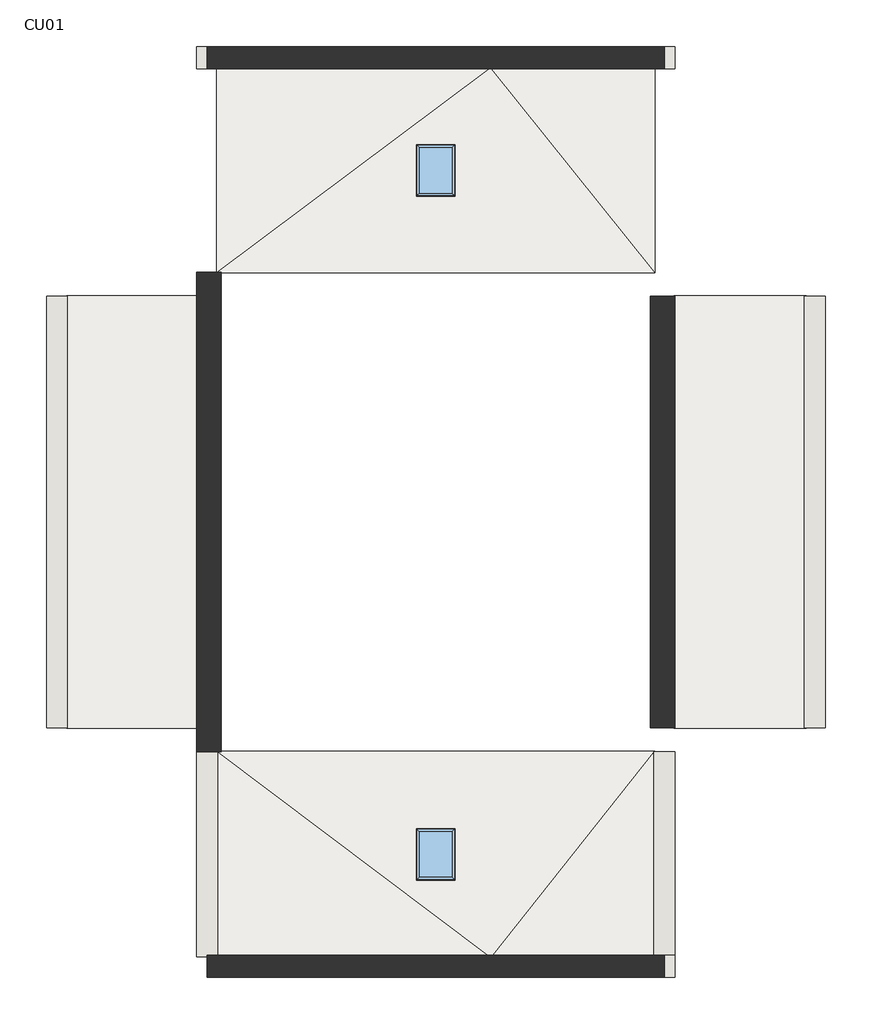
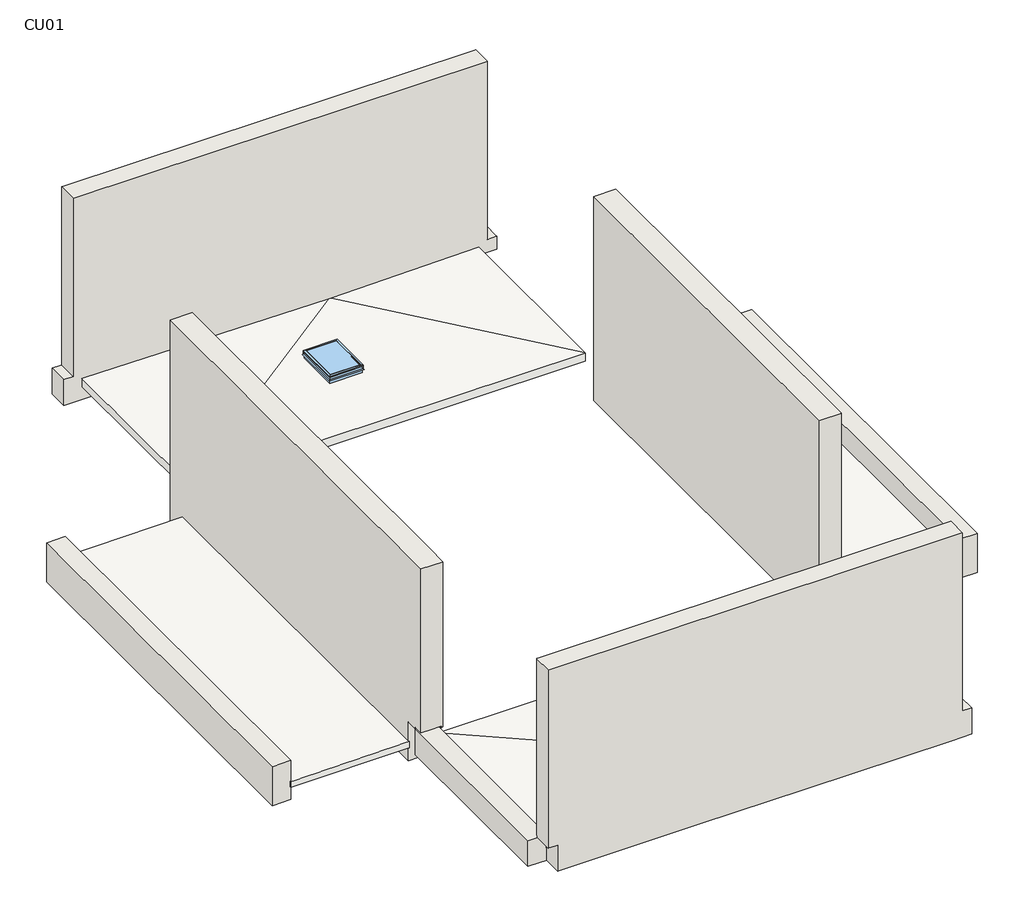
# One storey: 8 walls, 4 roofs, 2 windows.
"""IFC4 building model written with IfcOpenShell, lengths in millimetres."""

import ifcopenshell
import ifcopenshell.guid

model = None  # the IFC model being written
_history = None  # IfcOwnerHistory: only IFC2X3 demands one
_inside = {}  # id of a spatial element -> (the spatial element, [elements in it])
_under = {}  # id of a project, library or spatial element -> (it, [spatial elements below it])
_declared = {}  # id of a project -> (the project, [libraries it declares])
_typed = {}  # id of a type object -> (the type object, [elements of that type])
_made_of = {}  # id of a material, layer set ... -> (it, [elements and type objects made of it])


def new_model(schema):
    """Start an empty IFC model of exactly this schema.

    Asked for "IFC4X3", IfcOpenShell would pick the latest addendum, in which some entities
    have other attributes; the version numbers below select the first issue.
    IFC2X3 requires an IfcOwnerHistory on every rooted entity: one is made here for all.
    """
    global model, _history
    if schema == "IFC4X3":
        model = ifcopenshell.file(schema_version=(4, 3, 0, 0))
    else:
        model = ifcopenshell.file(schema=schema)
    _inside.clear()
    _under.clear()
    _declared.clear()
    _typed.clear()
    _made_of.clear()
    _history = None
    if model.schema == "IFC2X3":
        org = make("IfcOrganization", Name="unknown")
        user = make(
            "IfcPersonAndOrganization",
            ThePerson=make("IfcPerson", FamilyName="unknown"),
            TheOrganization=org,
        )
        app = make(
            "IfcApplication",
            ApplicationDeveloper=org,
            Version="unknown",
            ApplicationFullName="unknown",
            ApplicationIdentifier="unknown",
        )
        _history = make(
            "IfcOwnerHistory",
            OwningUser=user,
            OwningApplication=app,
            ChangeAction="ADDED",
            CreationDate=0,
        )
    return model


def make(cls, **values):
    """One entity of the class cls with the attributes given. An attribute that is None is left unset."""
    return model.create_entity(
        cls, **{name: value for name, value in values.items() if value is not None}
    )


def rooted(cls, **values):
    """An entity with a GlobalId (a new one), such as an element, a storey or a relation."""
    return make(cls, GlobalId=ifcopenshell.guid.new(), OwnerHistory=_history, **values)


def si_unit(unit_type, name, prefix=None):
    """IfcSIUnit, for example si_unit("LENGTHUNIT", "METRE", prefix="MILLI")."""
    return make("IfcSIUnit", UnitType=unit_type, Prefix=prefix, Name=name)


def assignment(units):
    """IfcUnitAssignment: the units of a project."""
    return None if units is None else make("IfcUnitAssignment", Units=units)


def point(xyz):
    """IfcCartesianPoint."""
    return None if xyz is None else make("IfcCartesianPoint", Coordinates=xyz)


def direction(xyz):
    """IfcDirection."""
    return None if xyz is None else make("IfcDirection", DirectionRatios=xyz)


def frame(location, z_axis=None, x_axis=None):
    """IfcAxis2Placement3D, a coordinate frame: its origin and axes. An axis left out is left unset."""
    return make(
        "IfcAxis2Placement3D",
        Location=point(location),
        Axis=direction(z_axis),
        RefDirection=direction(x_axis),
    )


def origin():
    """The frame at (0, 0, 0) with its axes left unset."""
    return frame((0.0, 0.0, 0.0))


def place(relative_to, where):
    """IfcLocalPlacement: puts the frame where relative to a parent placement (None: the world)."""
    return make(
        "IfcLocalPlacement", PlacementRelTo=relative_to, RelativePlacement=where
    )


def context(
    kind, dimensions, precision=None, world=None, true_north=None, identifier=None
):
    """IfcGeometricRepresentationContext, for example the 3D "Model" context."""
    return make(
        "IfcGeometricRepresentationContext",
        ContextIdentifier=identifier,
        ContextType=kind,
        CoordinateSpaceDimension=dimensions,
        Precision=precision,
        WorldCoordinateSystem=world,
        TrueNorth=true_north,
    )


def project(units=None, contexts=None):
    """IfcProject with its units and contexts."""
    return rooted(
        "IfcProject",
        Name="project",
        RepresentationContexts=contexts,
        UnitsInContext=assignment(units),
    )


def spatial(cls, under=None, at=None, **own):
    """A site, building, storey or space (cls), placed at a placement, below another one or the project."""
    s = rooted(cls, ObjectPlacement=at, **own)
    if under is not None:
        _under.setdefault(under.id(), (under, []))[1].append(s)
    return s


def polyline(points):
    """IfcPolyline through the points."""
    return make("IfcPolyline", Points=[point(p) for p in points])


def circle_curve(where, radius):
    """IfcCircle in the frame where."""
    return make("IfcCircle", Position=where, Radius=radius)


def outline(outer, holes=None, kind="AREA"):
    """IfcArbitraryClosedProfileDef: a profile drawn as a closed curve; with holes, ...WithVoids."""
    if holes is None:
        return make("IfcArbitraryClosedProfileDef", ProfileType=kind, OuterCurve=outer)
    return make(
        "IfcArbitraryProfileDefWithVoids",
        ProfileType=kind,
        OuterCurve=outer,
        InnerCurves=holes,
    )


def extrude(swept, where, along, depth):
    """IfcExtrudedAreaSolid: the profile swept, set in the frame where, extruded along a direction by depth."""
    return make(
        "IfcExtrudedAreaSolid",
        SweptArea=swept,
        Position=where,
        ExtrudedDirection=direction(along),
        Depth=depth,
    )


def faces_of(points, faces, orient=None, outer=None):
    """IfcFace entities. A face is a list of loops; a loop is a list of indices into points, from 0.

    orient and outer hold one flag for each loop. By default every Orientation is true, the
    first loop of a face is its IfcFaceOuterBound and the others are IfcFaceBound.
    """
    made = []
    for i, loops in enumerate(faces):
        bounds = []
        for j, loop in enumerate(loops):
            is_outer = j == 0 if outer is None else outer[i][j]
            bounds.append(
                make(
                    "IfcFaceOuterBound" if is_outer else "IfcFaceBound",
                    Bound=make("IfcPolyLoop", Polygon=[points[k] for k in loop]),
                    Orientation=True if orient is None else orient[i][j],
                )
            )
        made.append(make("IfcFace", Bounds=bounds))
    return made


def faceted_brep(points, faces, orient=None, outer=None, voids=None):
    """IfcFacetedBrep: a solid bounded by flat faces; with voids (closed shells), ...WithVoids."""
    shared = [point(p) for p in points]
    hull = make("IfcClosedShell", CfsFaces=faces_of(shared, faces, orient, outer))
    if voids is None:
        return make("IfcFacetedBrep", Outer=hull)
    return make(
        "IfcFacetedBrepWithVoids",
        Outer=hull,
        Voids=[
            make(cls, CfsFaces=faces_of(shared, fs, o, b)) for cls, fs, o, b in voids
        ],
    )


def shape(context_of_items, identifier, shape_type, items):
    """IfcShapeRepresentation: the items that make up one representation, for example the "Body"."""
    return make(
        "IfcShapeRepresentation",
        ContextOfItems=context_of_items,
        RepresentationIdentifier=identifier,
        RepresentationType=shape_type,
        Items=items,
    )


def source(mapping_origin, context_of_items, identifier, shape_type, items):
    """IfcRepresentationMap: a shape defined once, which mapped items show again and again."""
    return make(
        "IfcRepresentationMap",
        MappingOrigin=mapping_origin,
        MappedRepresentation=shape(context_of_items, identifier, shape_type, items),
    )


def transform(
    local_origin,
    x_axis=None,
    y_axis=None,
    z_axis=None,
    scale=None,
    scale2=None,
    scale3=None,
    uniform=True,
):
    """IfcCartesianTransformationOperator3D, or its non-uniform kind. x_axis, y_axis, z_axis: its Axis1, 2, 3."""
    if uniform:
        return make(
            "IfcCartesianTransformationOperator3D",
            Axis1=direction(x_axis),
            Axis2=direction(y_axis),
            LocalOrigin=point(local_origin),
            Scale=scale,
            Axis3=direction(z_axis),
        )
    return make(
        "IfcCartesianTransformationOperator3DnonUniform",
        Axis1=direction(x_axis),
        Axis2=direction(y_axis),
        LocalOrigin=point(local_origin),
        Scale=scale,
        Axis3=direction(z_axis),
        Scale2=scale2,
        Scale3=scale3,
    )


def mapped(mapping_source, mapping_target):
    """IfcMappedItem: shows the shape of a source again, moved by a transform."""
    return make(
        "IfcMappedItem", MappingSource=mapping_source, MappingTarget=mapping_target
    )


def made_of(thing, what):
    """Note that an element or type object is made of a material, layer set ...; save() writes the relation."""
    if what is not None:
        _made_of.setdefault(what.id(), (what, []))[1].append(thing)
    return thing


def element(
    cls,
    number,
    at=None,
    inside=None,
    cuts=None,
    type_object=None,
    material=None,
    context=None,
    identifier="Body",
    shape_type=None,
    held_by="IfcProductDefinitionShape",
    body=None,
    shapes=None,
    **own,
):
    """One element of the class cls, such as IfcWall. Its Tag is "e" and its number.

    at: its placement. inside: the storey or other place that contains it. cuts: it is an
    opening in that element (IfcRelVoidsElement). A single representation is given by context,
    identifier, shape_type and body (its items); several are given by shapes. held_by: the class
    of the entity that holds the representations. save() writes the other relations.
    """
    e = rooted(cls, Tag="e%d" % number, ObjectPlacement=at, **own)
    if body is not None:
        shapes = [shape(context, identifier, shape_type, body)]
    if shapes is not None:
        e.Representation = make(held_by, Representations=shapes)
    if inside is not None:
        _inside.setdefault(inside.id(), (inside, []))[1].append(e)
    if cuts is not None:
        rooted(
            "IfcRelVoidsElement", RelatingBuildingElement=cuts, RelatedOpeningElement=e
        )
    if type_object is not None:
        _typed.setdefault(type_object.id(), (type_object, []))[1].append(e)
    return made_of(e, material)


def aggregate(whole, parts):
    """IfcRelAggregates: a whole, such as a stair, and the parts it consists of."""
    return rooted("IfcRelAggregates", RelatingObject=whole, RelatedObjects=parts)


def save(model, path):
    """Write the relations noted so far, then the file.

    IfcRelAggregates (storeys below a building ...), IfcRelContainedInSpatialStructure (elements
    in a storey), IfcRelDefinesByType, IfcRelAssociatesMaterial and IfcRelDeclares: one each for
    every whole, place, type object, material and project.
    """
    for whole, parts in _under.values():
        aggregate(whole, parts)
    for where, things in _inside.values():
        rooted(
            "IfcRelContainedInSpatialStructure",
            RelatedElements=things,
            RelatingStructure=where,
        )
    for kind, things in _typed.values():
        rooted("IfcRelDefinesByType", RelatedObjects=things, RelatingType=kind)
    for what, things in _made_of.values():
        rooted("IfcRelAssociatesMaterial", RelatedObjects=things, RelatingMaterial=what)
    for by, libraries in _declared.values():
        rooted("IfcRelDeclares", RelatingContext=by, RelatedDefinitions=libraries)
    model.write(path)


def plane_surface(at):
    """IfcPlane: the flat surface through the origin of the frame at, square to its z axis."""
    return make("IfcPlane", Position=at)


def cylinder_surface(at, radius):
    """IfcCylindricalSurface: all points at the distance radius from the z axis of the frame at."""
    return make("IfcCylindricalSurface", Position=at, Radius=radius)


def advanced_brep(points, edges, surfaces, faces):
    """IfcAdvancedBrep: a solid bounded by faces that lie on surfaces and meet in shared edges.

    An edge is (start, end): straight between two places in points (the first is 0);
    or (start, end, curve); or (start, end, curve, False) where it runs against its curve.
    A face is (place in surfaces, loops), or (place, loops, False) where it looks against
    its surface's normal. A loop lists edges by number (the first is 1), with a minus sign
    where the edge is run from its end to its start. The first loop is the outer one.
    """
    corners = [point(p) for p in points]
    vertices = [make("IfcVertexPoint", VertexGeometry=c) for c in corners]
    made = []
    for start, end, *more in edges:
        made.append(
            make(
                "IfcEdgeCurve",
                EdgeStart=vertices[start],
                EdgeEnd=vertices[end],
                EdgeGeometry=more[0] if more else make("IfcPolyline", Points=[corners[start], corners[end]]),
                SameSense=more[1] if len(more) > 1 else True,
            )
        )
    hull = []
    for where, loops, *sense in faces:
        bounds = []
        for j, loop in enumerate(loops):
            ring = [make("IfcOrientedEdge", EdgeElement=made[abs(k) - 1], Orientation=k > 0) for k in loop]
            bounds.append(
                make(
                    "IfcFaceOuterBound" if j == 0 else "IfcFaceBound",
                    Bound=make("IfcEdgeLoop", EdgeList=ring),
                    Orientation=True,
                )
            )
        hull.append(make("IfcAdvancedFace", Bounds=bounds, FaceSurface=surfaces[where], SameSense=sense[0] if sense else True))
    return make("IfcAdvancedBrep", Outer=make("IfcClosedShell", CfsFaces=hull))


def claraboya_0711_x_0965mm_26b2130f(model_context):
    return source(origin(), model_context, "Body", "SolidModel", [
        faceted_brep([(254.440073, 370.1040988, 4001.2), (279.840073, 395.5040988, 4001.2), (279.840073, -569.4959012, 4001.2), (254.440073, -544.0959012, 4001.2), (254.440073, 370.1040988, 4026.6), (254.440073, -544.0959012, 4026.6), (292.540073, 408.2040988, 4026.6), (292.540073, -582.1959012, 4026.6), (292.540073, 408.2040988, 4001.2), (292.540073, -582.1959012, 4001.2), (292.540073, 408.2040988, 3950.4), (292.540073, -582.1959012, 3950.4), (307.1089145, 422.7729403, 3929.5935381), (307.1089145, -596.7647427, 3929.5935381), (301.907299, 417.5713248, 3925.9513277), (301.907299, -591.5631272, 3925.9513277), (286.190073, 401.8540988, 3948.3978527), (286.190073, -575.8459012, 3948.3978527), (286.190073, 401.8540988, 4001.2), (286.190073, -575.8459012, 4001.2), (-431.159927, -569.4959012, 4001.2), (-405.759927, -544.0959012, 4001.2), (-405.759927, -544.0959012, 4026.6), (-443.859927, -582.1959012, 4026.6), (-443.859927, -582.1959012, 4001.2), (-443.859927, -582.1959012, 3950.4), (-458.4287685, -596.7647427, 3929.5935381), (-453.227153, -591.5631272, 3925.9513277), (-437.509927, -575.8459012, 3948.3978527), (-437.509927, -575.8459012, 4001.2), (-431.159927, 395.5040988, 4001.2), (-405.759927, 370.1040988, 4001.2), (-405.759927, 370.1040988, 4026.6), (-443.859927, 408.2040988, 4026.6), (-443.859927, 408.2040988, 4001.2), (-443.859927, 408.2040988, 3950.4), (-458.4287685, 422.7729403, 3929.5935381), (-453.227153, 417.5713248, 3925.9513277), (-437.509927, 401.8540988, 3948.3978527), (-437.509927, 401.8540988, 4001.2)], [[[0, 1, 2, 3]], [[4, 0, 3, 5]], [[6, 4, 5, 7]], [[8, 6, 7, 9]], [[10, 8, 9, 11]], [[12, 10, 11, 13]], [[14, 12, 13, 15]], [[16, 14, 15, 17]], [[18, 16, 17, 19]], [[1, 18, 19, 2]], [[3, 2, 20, 21]], [[5, 3, 21, 22]], [[7, 5, 22, 23]], [[9, 7, 23, 24]], [[11, 9, 24, 25]], [[13, 11, 25, 26]], [[15, 13, 26, 27]], [[17, 15, 27, 28]], [[19, 17, 28, 29]], [[2, 19, 29, 20]], [[21, 20, 30, 31]], [[22, 21, 31, 32]], [[23, 22, 32, 33]], [[24, 23, 33, 34]], [[25, 24, 34, 35]], [[26, 25, 35, 36]], [[27, 26, 36, 37]], [[28, 27, 37, 38]], [[29, 28, 38, 39]], [[20, 29, 39, 30]], [[31, 30, 1, 0]], [[32, 31, 0, 4]], [[33, 32, 4, 6]], [[34, 33, 6, 8]], [[35, 34, 8, 10]], [[36, 35, 10, 12]], [[37, 36, 12, 14]], [[38, 37, 14, 16]], [[39, 38, 16, 18]], [[30, 39, 18, 1]]]),
        faceted_brep([(279.840073, -569.4959012, 4001.2), (279.840073, -569.4959012, 3848.8), (279.840073, 395.5040988, 3848.8), (279.840073, 395.5040988, 4001.2), (254.440073, -544.0959012, 4001.2), (254.440073, 370.1040988, 4001.2), (254.440073, -544.0959012, 3975.8), (254.440073, 370.1040988, 3975.8), (235.390073, -525.0459012, 3975.8), (235.390073, 351.0540988, 3975.8), (235.390073, -525.0459012, 3848.8), (235.390073, 351.0540988, 3848.8), (-431.159927, 395.5040988, 3848.8), (-431.159927, 395.5040988, 4001.2), (-405.759927, 370.1040988, 4001.2), (-405.759927, 370.1040988, 3975.8), (-386.709927, 351.0540988, 3975.8), (-386.709927, 351.0540988, 3848.8), (-431.159927, -569.4959012, 3848.8), (-431.159927, -569.4959012, 4001.2), (-405.759927, -544.0959012, 4001.2), (-405.759927, -544.0959012, 3975.8), (-386.709927, -525.0459012, 3975.8), (-386.709927, -525.0459012, 3848.8)], [[[0, 1, 2, 3]], [[4, 0, 3, 5]], [[6, 4, 5, 7]], [[8, 6, 7, 9]], [[10, 8, 9, 11]], [[1, 10, 11, 2]], [[3, 2, 12, 13]], [[5, 3, 13, 14]], [[7, 5, 14, 15]], [[9, 7, 15, 16]], [[11, 9, 16, 17]], [[2, 11, 17, 12]], [[13, 12, 18, 19]], [[14, 13, 19, 20]], [[15, 14, 20, 21]], [[16, 15, 21, 22]], [[17, 16, 22, 23]], [[12, 17, 23, 18]], [[19, 18, 1, 0]], [[20, 19, 0, 4]], [[21, 20, 4, 6]], [[22, 21, 6, 8]], [[23, 22, 8, 10]], [[18, 23, 10, 1]]]),
        extrude(outline(polyline([(254.440073, -544.0959012), (-405.759927, -544.0959012), (-405.759927, 370.1040988), (254.440073, 370.1040988), (254.440073, -544.0959012)])), frame((0.0, 0.0, 4020.25), z_axis=(0.0, 0.0, 1.0), x_axis=(1.0, 0.0, 0.0)), (0.0, 0.0, 1.0), 6.35),
    ])


def claraboya_0711_x_0965mm_17ef4467(model_context):
    return source(origin(), model_context, "Body", "SolidModel", [
        faceted_brep([(254.440073, -370.1040988, 4001.2), (254.440073, 544.0959012, 4001.2), (279.840073, 569.4959012, 4001.2), (279.840073, -395.5040988, 4001.2), (254.440073, -370.1040988, 4026.6), (254.440073, 544.0959012, 4026.6), (292.540073, -408.2040988, 4026.6), (292.540073, 582.1959012, 4026.6), (292.540073, -408.2040988, 4001.2), (292.540073, 582.1959012, 4001.2), (292.540073, -408.2040988, 3950.4), (292.540073, 582.1959012, 3950.4), (307.1089145, -422.7729403, 3929.5935381), (307.1089145, 596.7647427, 3929.5935381), (301.907299, -417.5713248, 3925.9513277), (301.907299, 591.5631272, 3925.9513277), (286.190073, -401.8540988, 3948.3978527), (286.190073, 575.8459012, 3948.3978527), (286.190073, -401.8540988, 4001.2), (286.190073, 575.8459012, 4001.2), (-405.759927, 544.0959012, 4001.2), (-431.159927, 569.4959012, 4001.2), (-405.759927, 544.0959012, 4026.6), (-443.859927, 582.1959012, 4026.6), (-443.859927, 582.1959012, 4001.2), (-443.859927, 582.1959012, 3950.4), (-458.4287685, 596.7647427, 3929.5935381), (-453.227153, 591.5631272, 3925.9513277), (-437.509927, 575.8459012, 3948.3978527), (-437.509927, 575.8459012, 4001.2), (-405.759927, -370.1040988, 4001.2), (-431.159927, -395.5040988, 4001.2), (-405.759927, -370.1040988, 4026.6), (-443.859927, -408.2040988, 4026.6), (-443.859927, -408.2040988, 4001.2), (-443.859927, -408.2040988, 3950.4), (-458.4287685, -422.7729403, 3929.5935381), (-453.227153, -417.5713248, 3925.9513277), (-437.509927, -401.8540988, 3948.3978527), (-437.509927, -401.8540988, 4001.2)], [[[0, 1, 2, 3]], [[4, 5, 1, 0]], [[6, 7, 5, 4]], [[8, 9, 7, 6]], [[10, 11, 9, 8]], [[12, 13, 11, 10]], [[14, 15, 13, 12]], [[16, 17, 15, 14]], [[18, 19, 17, 16]], [[3, 2, 19, 18]], [[1, 20, 21, 2]], [[5, 22, 20, 1]], [[7, 23, 22, 5]], [[9, 24, 23, 7]], [[11, 25, 24, 9]], [[13, 26, 25, 11]], [[15, 27, 26, 13]], [[17, 28, 27, 15]], [[19, 29, 28, 17]], [[2, 21, 29, 19]], [[20, 30, 31, 21]], [[22, 32, 30, 20]], [[23, 33, 32, 22]], [[24, 34, 33, 23]], [[25, 35, 34, 24]], [[26, 36, 35, 25]], [[27, 37, 36, 26]], [[28, 38, 37, 27]], [[29, 39, 38, 28]], [[21, 31, 39, 29]], [[30, 0, 3, 31]], [[32, 4, 0, 30]], [[33, 6, 4, 32]], [[34, 8, 6, 33]], [[35, 10, 8, 34]], [[36, 12, 10, 35]], [[37, 14, 12, 36]], [[38, 16, 14, 37]], [[39, 18, 16, 38]], [[31, 3, 18, 39]]]),
        faceted_brep([(279.840073, 569.4959012, 4001.2), (279.840073, -395.5040988, 4001.2), (279.840073, -395.5040988, 3848.8), (279.840073, 569.4959012, 3848.8), (254.440073, 544.0959012, 4001.2), (254.440073, -370.1040988, 4001.2), (254.440073, 544.0959012, 3975.8), (254.440073, -370.1040988, 3975.8), (235.390073, 525.0459012, 3975.8), (235.390073, -351.0540988, 3975.8), (235.390073, 525.0459012, 3848.8), (235.390073, -351.0540988, 3848.8), (-431.159927, -395.5040988, 4001.2), (-431.159927, -395.5040988, 3848.8), (-405.759927, -370.1040988, 4001.2), (-405.759927, -370.1040988, 3975.8), (-386.709927, -351.0540988, 3975.8), (-386.709927, -351.0540988, 3848.8), (-431.159927, 569.4959012, 4001.2), (-431.159927, 569.4959012, 3848.8), (-405.759927, 544.0959012, 4001.2), (-405.759927, 544.0959012, 3975.8), (-386.709927, 525.0459012, 3975.8), (-386.709927, 525.0459012, 3848.8)], [[[0, 1, 2, 3]], [[4, 5, 1, 0]], [[6, 7, 5, 4]], [[8, 9, 7, 6]], [[10, 11, 9, 8]], [[3, 2, 11, 10]], [[1, 12, 13, 2]], [[5, 14, 12, 1]], [[7, 15, 14, 5]], [[9, 16, 15, 7]], [[11, 17, 16, 9]], [[2, 13, 17, 11]], [[12, 18, 19, 13]], [[14, 20, 18, 12]], [[15, 21, 20, 14]], [[16, 22, 21, 15]], [[17, 23, 22, 16]], [[13, 19, 23, 17]], [[18, 0, 3, 19]], [[20, 4, 0, 18]], [[21, 6, 4, 20]], [[22, 8, 6, 21]], [[23, 10, 8, 22]], [[19, 3, 10, 23]]]),
        extrude(outline(polyline([(254.440073, 544.0959012), (254.440073, -370.1040988), (-405.759927, -370.1040988), (-405.759927, 544.0959012), (254.440073, 544.0959012)])), frame((0.0, 0.0, 4020.25), z_axis=(0.0, 0.0, 1.0), x_axis=(1.0, 0.0, 0.0)), (0.0, 0.0, 1.0), 6.35),
    ])


model = new_model("IFC4")

# Units and contexts
model_context = context("Model", 3, world=origin())
ifc_project = project(units=[si_unit("LENGTHUNIT", "METRE", prefix="MILLI")], contexts=[model_context])

# Site, building, storey
site = spatial("IfcSite", under=ifc_project)
building = spatial("IfcBuilding", under=site)
storey = spatial("IfcBuildingStorey", under=building, Name="CU01", Elevation=2430.0)

# Roofs
placement = place(None, origin())
element("IfcRoof", 1, ObjectType="ACAB CUB GRAVA INF-A_PABLO", at=placement, inside=storey, context=model_context, shape_type="Brep", body=[
    faceted_brep([(-12165.0, -4267.5, 2730.0), (-12165.0, -4252.5, 2730.0), (-12165.0, -232.5, 2730.0), (-12165.0, -217.5, 2730.0), (-12165.0, -217.5, 2921.2), (-12165.0, -232.5, 2921.2), (-12165.0, -4252.5, 2921.2), (-12165.0, -4267.5, 2921.2), (-12235.0, -217.5, 2730.0), (-20835.0, -217.5, 2730.0), (-20835.0, -217.5, 2921.2), (-15415.0, -217.5, 2871.2), (-16188.95, -1804.45, 2890.7919753), (-16188.95, -1804.45, 2730.0), (-16188.95, -2680.55, 2730.0), (-16188.95, -2680.55, 2901.6080247), (-16811.05, -2680.55, 2730.0), (-16811.05, -2680.55, 2901.6080247), (-16811.05, -1804.45, 2730.0), (-16811.05, -1804.45, 2890.7919753), (-20750.0, -4267.5, 2730.0), (-20835.0, -4267.5, 2730.0), (-20835.0, -4252.5, 2730.0), (-20835.0, -232.5, 2730.0), (-20835.0, -4267.5, 2921.2), (-20835.0, -4252.5, 2921.2), (-20835.0, -232.5, 2921.2), (-20750.0, -4267.5, 2921.2), (-12177.037037, -4252.5, 2921.0148148), (-12180.0, -4248.8076923, 2920.9692308), (-15402.962963, -232.5, 2871.3851852), (-15435.0740741, -232.5, 2871.3851852)], [[[0, 1, 2, 3, 4, 5, 6, 7]], [[3, 8, 9, 10, 11, 4]], [[12, 13, 14, 15]], [[15, 14, 16, 17]], [[17, 16, 18, 19]], [[13, 12, 19, 18]], [[3, 2, 1, 0, 20, 21, 22, 23, 9, 8], [14, 13, 18, 16]], [[9, 23, 22, 21, 24, 25, 26, 10]], [[0, 7, 27, 24, 21, 20]], [[24, 27, 7, 28, 29, 30, 11, 31], [12, 15, 17, 19]], [[7, 6, 5, 4, 11, 30, 29, 28]], [[10, 26, 25, 24, 31, 11]]]),
])
element("IfcRoof", 2, ObjectType="ACAB CUB GRAVA INF-B_PABLO", at=placement, inside=storey, context=model_context, shape_type="Brep", body=[
    faceted_brep([(-23810.0, -4717.5, 2430.0), (-21230.0, -4717.5, 2430.0), (-21215.0, -4717.5, 2430.0), (-21215.0, -13267.5, 2430.0), (-21215.0, -13282.5, 2430.0), (-21230.0, -13282.5, 2430.0), (-23810.0, -13282.5, 2430.0), (-23810.0, -13267.5, 2430.0), (-23810.0, -4732.5, 2430.0), (-21215.0, -4717.5, 2581.2), (-23810.0, -4717.5, 2551.2), (-21230.0, -4717.5, 2581.0265896), (-23810.0, -13282.5, 2551.2), (-23810.0, -13267.5, 2551.2), (-23810.0, -9000.0, 2551.2), (-23810.0, -4732.5, 2551.2), (-21215.0, -13282.5, 2581.2), (-21215.0, -13267.5, 2581.2)], [[[0, 1, 2, 3, 4, 5, 6, 7, 8]], [[9, 2, 1, 0, 10, 11]], [[10, 0, 8, 7, 6, 12, 13, 14, 15]], [[12, 6, 5, 4, 16]], [[10, 15, 14, 13, 12, 16, 17, 9, 11]], [[16, 4, 3, 2, 9, 17]]]),
])
element("IfcRoof", 3, ObjectType="ACAB CUB GRAVA INF-A_PABLO", at=placement, inside=storey, context=model_context, shape_type="Brep", body=[
    faceted_brep([(-12165.0, -17812.5, 2730.0), (-12165.0, -17767.5, 2730.0), (-12165.0, -13747.5, 2730.0), (-12165.0, -13732.5, 2730.0), (-12165.0, -13732.5, 2921.2), (-12165.0, -13747.5, 2921.2), (-12165.0, -17767.5, 2921.2), (-12165.0, -17812.5, 2921.2), (-15405.0, -17812.5, 2871.2), (-20820.0, -17812.5, 2921.0618785), (-20835.0, -17812.5, 2921.2), (-20835.0, -17812.5, 2730.0), (-20820.0, -17812.5, 2730.0), (-16188.95, -16210.55, 2730.0), (-16188.95, -16210.55, 2890.8317402), (-16188.95, -15334.45, 2901.5682598), (-16188.95, -15334.45, 2730.0), (-16811.05, -15334.45, 2901.5682598), (-16811.05, -15334.45, 2730.0), (-16811.05, -16210.55, 2890.8317402), (-16811.05, -16210.55, 2730.0), (-20835.0, -17797.5, 2730.0), (-20835.0, -13732.5, 2730.0), (-20820.0, -13732.5, 2730.0), (-20750.0, -13732.5, 2730.0), (-20835.0, -17797.5, 2921.2), (-20835.0, -13732.5, 2921.2), (-20820.0, -13732.5, 2921.2), (-20750.0, -13732.5, 2921.2), (-12176.9117647, -13747.5, 2921.0161765), (-12180.0, -13751.3888889, 2920.9685185), (-15369.2647059, -17767.5, 2871.7514706), (-20820.0, -13743.7707182, 2921.0618785), (-15464.8897059, -17767.5, 2871.7514706)], [[[0, 1, 2, 3, 4, 5, 6, 7]], [[0, 7, 8, 9, 10, 11, 12]], [[13, 14, 15, 16]], [[16, 15, 17, 18]], [[18, 17, 19, 20]], [[14, 13, 20, 19]], [[3, 2, 1, 0, 12, 11, 21, 22, 23, 24], [13, 16, 18, 20]], [[22, 21, 11, 10, 25, 26]], [[4, 3, 24, 23, 22, 26, 27, 28]], [[7, 6, 5, 4, 29, 30, 31, 8]], [[4, 28, 27, 26, 32, 33, 8, 31, 30, 29], [15, 14, 19, 17]], [[26, 25, 10, 9, 8, 33, 32]]]),
])
element("IfcRoof", 4, ObjectType="ACAB CUB GRAVA INF-B_PABLO", at=placement, inside=storey, context=model_context, shape_type="Brep", body=[
    faceted_brep([(-11785.0, -4717.5, 2430.0), (-9165.0, -4717.5, 2430.0), (-9165.0, -4732.5, 2430.0), (-9165.0, -13267.5, 2430.0), (-9165.0, -13282.5, 2430.0), (-11785.0, -13282.5, 2430.0), (-11785.0, -13267.5, 2430.0), (-11785.0, -4732.5, 2430.0), (-9165.0, -4717.5, 2551.2), (-11785.0, -4717.5, 2581.2), (-9165.0, -13282.5, 2551.2), (-9165.0, -4732.5, 2551.2), (-9165.0, -9000.0, 2551.2), (-9165.0, -13267.5, 2551.2), (-11785.0, -13282.5, 2581.2), (-11785.0, -4732.5, 2581.2), (-11785.0, -13267.5, 2581.2)], [[[0, 1, 2, 3, 4, 5, 6, 7]], [[8, 1, 0, 9]], [[10, 4, 3, 2, 1, 8, 11, 12, 13]], [[14, 5, 4, 10]], [[12, 11, 8, 9, 15, 16, 14, 10, 13]], [[9, 0, 7, 6, 5, 14, 16, 15]]]),
])

# Walls
element("IfcWall", 5, ObjectType="MURO TIPO 1_EXTERIOR_PETO_PABLO", at=placement, inside=storey, context=model_context, shape_type="Brep", body=[
    faceted_brep([(-23795.0, -13267.5, 2130.0), (-23795.0, -4732.5, 2130.0), (-23795.0, -4732.5, 2430.0), (-23795.0, -13267.5, 2430.0), (-23795.0, -4732.5, 3030.0), (-23795.0, -13267.5, 3030.0), (-23795.0, -13267.5, 2551.3734104), (-23795.0, -4732.5, 2551.3734104), (-24205.0, -4732.5, 2130.0), (-24205.0, -13267.5, 2130.0), (-24205.0, -13267.5, 3030.0), (-24205.0, -4732.5, 3030.0), (-23810.0, -13267.5, 2430.0), (-23810.0, -13267.5, 2551.2), (-23810.0, -4732.5, 2551.2), (-23810.0, -4732.5, 2430.0), (-23810.0, -9000.0, 2551.2)], [[[0, 1, 2, 3]], [[4, 5, 6, 7]], [[8, 9, 10, 11]], [[1, 0, 9, 8]], [[5, 4, 11, 10]], [[5, 10, 9, 0, 3, 12, 13, 6]], [[1, 8, 11, 4, 7, 14, 15, 2]], [[15, 12, 3, 2]], [[12, 15, 14, 16, 13]], [[13, 16, 14, 7, 6]]]),
])
element("IfcWall", 6, ObjectType="MURO TIPO 1_EXTERIOR_PETO_PABLO", at=placement, inside=storey, context=model_context, shape_type="Brep", body=[
    faceted_brep([(-8795.0, -13267.5, 2130.0), (-8795.0, -4732.5, 2130.0), (-8795.0, -4732.5, 3030.0), (-8795.0, -13267.5, 3030.0), (-9205.0, -4732.5, 2130.0), (-9205.0, -13267.5, 2130.0), (-9205.0, -13267.5, 2430.0), (-9205.0, -4732.5, 2430.0), (-9205.0, -13267.5, 3030.0), (-9205.0, -4732.5, 3030.0), (-9205.0, -4732.5, 2551.6580153), (-9205.0, -13267.5, 2551.6580153), (-9165.0, -13267.5, 2551.2), (-9165.0, -13267.5, 2430.0), (-9165.0, -4732.5, 2430.0), (-9165.0, -4732.5, 2551.2), (-9165.0, -9000.0, 2551.2)], [[[0, 1, 2, 3]], [[4, 5, 6, 7]], [[8, 9, 10, 11]], [[1, 0, 5, 4]], [[3, 2, 9, 8]], [[0, 3, 8, 11, 12, 13, 6, 5]], [[2, 1, 4, 7, 14, 15, 10, 9]], [[13, 14, 7, 6]], [[14, 13, 12, 16, 15]], [[16, 12, 11, 10, 15]]]),
])
element("IfcWall", 7, ObjectType="MURO TIPO 1_EXTERIOR_PETO-CUB_PABLO", at=placement, inside=storey, context=model_context, shape_type="Brep", body=[
    faceted_brep([(-21230.0, -232.5, 2430.0), (-12235.0, -232.5, 2430.0), (-12235.0, -232.5, 2730.0), (-20835.0, -232.5, 2730.0), (-20835.0, -232.5, 2921.2), (-15435.0740741, -232.5, 2871.3851852), (-15402.962963, -232.5, 2871.3851852), (-12180.0, -232.5, 2920.9692308), (-12165.0, -232.5, 2921.2), (-12165.0, -232.5, 2730.0), (-11770.0, -232.5, 2730.0), (-11770.0, -232.5, 3030.0), (-11975.0, -232.5, 3030.0), (-11975.0, -232.5, 7150.0), (-12002.5, -232.5, 7150.0), (-21010.0, -232.5, 7150.0), (-21025.0, -232.5, 7150.0), (-21025.0, -232.5, 3030.0), (-21230.0, -232.5, 3030.0), (-21230.0, -232.5, 2730.0), (-12235.0, 207.5, 2430.0), (-17710.0, 207.5, 2430.0), (-21230.0, 207.5, 2430.0), (-21230.0, 207.5, 3030.0), (-21025.0, 207.5, 3030.0), (-21025.0, 207.5, 7150.0), (-21010.0, 207.5, 7150.0), (-12002.5, 207.5, 7150.0), (-11975.0, 207.5, 7150.0), (-11975.0, 207.5, 3030.0), (-11770.0, 207.5, 3030.0), (-11770.0, 207.5, 2730.0), (-12235.0, 207.5, 2730.0), (-12165.0, -217.5, 2730.0), (-12235.0, -217.5, 2730.0), (-12165.0, -217.5, 2921.2), (-15415.0, -217.5, 2871.2), (-20835.0, -217.5, 2921.2), (-20835.0, -217.5, 2730.0), (-21230.0, 192.5, 3030.0), (-21230.0, -217.5, 3030.0), (-11770.0, -217.5, 3030.0), (-11770.0, 192.5, 3030.0)], [[[0, 1, 2, 3, 4, 5, 6, 7, 8, 9, 10, 11, 12, 13, 14, 15, 16, 17, 18, 19]], [[20, 21, 22, 23, 24, 25, 26, 27, 28, 29, 30, 31, 32]], [[1, 0, 22, 21, 20]], [[16, 15, 14, 13, 28, 27, 26, 25]], [[32, 31, 10, 9, 33, 34]], [[2, 1, 20, 32, 34]], [[33, 35, 36, 37, 38, 34]], [[35, 33, 9, 8]], [[34, 38, 3, 2]], [[38, 37, 4, 3]], [[16, 25, 24, 17]], [[17, 24, 23, 39, 40, 18]], [[22, 0, 19, 18, 40, 39, 23]], [[36, 35, 8, 7, 6]], [[37, 36, 5, 4]], [[36, 6, 5]], [[28, 13, 12, 29]], [[29, 12, 11, 41, 42, 30]], [[11, 10, 31, 30, 42, 41]]]),
])
element("IfcWall", 8, ObjectType="MURO TIPO 3B_ESTAR-EXT_YESO-CEMENTO_PABLO", at=placement, inside=storey, context=model_context, shape_type="Brep", body=[
    faceted_brep([(-12250.0, -4732.5, 2130.0), (-12250.0, -13267.5, 2130.0), (-12250.0, -13267.5, 6850.0), (-12250.0, -4732.5, 6850.0), (-11770.0, -13267.5, 2130.0), (-11770.0, -4732.5, 2130.0), (-11770.0, -4732.5, 2430.0), (-11770.0, -13267.5, 2430.0), (-11770.0, -4732.5, 6850.0), (-11770.0, -13267.5, 6850.0), (-11770.0, -13267.5, 2581.0282443), (-11770.0, -4732.5, 2581.0282443), (-11785.0, -13267.5, 2130.0), (-11785.0, -13267.5, 6850.0), (-11785.0, -4732.5, 2430.0), (-11785.0, -13267.5, 2430.0), (-11785.0, -13267.5, 2581.2), (-11785.0, -4732.5, 2581.2)], [[[0, 1, 2, 3]], [[4, 5, 6, 7]], [[8, 9, 10, 11]], [[1, 0, 5, 4, 12]], [[3, 2, 13, 9, 8]], [[14, 15, 7, 6]], [[16, 17, 11, 10]], [[15, 14, 17, 16]], [[1, 12, 4, 7, 15, 16, 10, 9, 13, 2]], [[5, 0, 3, 8, 11, 17, 14, 6]]]),
])
element("IfcWall", 9, ObjectType="MURO TIPO 1_EXTERIOR_PETO_PABLO", at=placement, inside=storey, context=model_context, shape_type="Brep", body=[
    faceted_brep([(-11770.0, -17767.5, 2430.0), (-11770.0, -13747.5, 2430.0), (-11770.0, -13747.5, 3030.0), (-11770.0, -17767.5, 3030.0), (-12180.0, -13747.5, 2430.0), (-12180.0, -17767.5, 2430.0), (-12180.0, -17767.5, 2730.0), (-12180.0, -13747.5, 2730.0), (-12180.0, -17767.5, 3030.0), (-12180.0, -13747.5, 3030.0), (-12180.0, -13747.5, 2921.0161765), (-12180.0, -13751.3888889, 2920.9685185), (-12180.0, -17767.5, 2920.9685185), (-11975.0, -17767.5, 3030.0), (-12165.0, -13747.5, 2921.2), (-12165.0, -13747.5, 2730.0), (-12165.0, -17767.5, 2730.0), (-12165.0, -17767.5, 2921.2), (-12176.9117647, -13747.5, 2921.0161765)], [[[0, 1, 2, 3]], [[4, 5, 6, 7]], [[8, 9, 10, 11, 12]], [[1, 0, 5, 4]], [[3, 2, 9, 8, 13]], [[14, 15, 16, 17]], [[7, 6, 16, 15]], [[11, 18, 14, 17, 12]], [[18, 11, 10]], [[2, 1, 4, 7, 15, 14, 18, 10, 9]], [[0, 3, 13, 8, 12, 17, 16, 6, 5]]]),
])
element("IfcWall", 10, ObjectType="MURO TIPO 1_EXTERIOR_PETO_PABLO", at=placement, inside=storey, context=model_context, shape_type="Brep", body=[
    faceted_brep([(-20820.0, -17797.5, 2430.0), (-20820.0, -17767.5, 2430.0), (-20820.0, -13537.5, 2430.0), (-20820.0, -13537.5, 3030.0), (-20820.0, -17767.5, 3030.0), (-20820.0, -17797.5, 3030.0), (-20820.0, -17797.5, 2921.0618785), (-20820.0, -17767.5, 2921.0618785), (-20820.0, -13743.7707182, 2921.0618785), (-20820.0, -13732.5, 2921.2), (-20820.0, -13732.5, 2730.0), (-20820.0, -17767.5, 2730.0), (-20820.0, -17797.5, 2730.0), (-21230.0, -13537.5, 2430.0), (-21230.0, -17797.5, 2430.0), (-21230.0, -17797.5, 3030.0), (-21230.0, -13537.5, 3030.0), (-21010.0, -17797.5, 3030.0), (-20835.0, -13732.5, 2730.0), (-20835.0, -17797.5, 2730.0), (-20835.0, -13732.5, 2921.2), (-20835.0, -17797.5, 2921.2)], [[[0, 1, 2, 3, 4, 5, 6, 7, 8, 9, 10, 11, 12]], [[13, 14, 15, 16]], [[2, 1, 0, 14, 13]], [[5, 4, 3, 16, 15, 17]], [[10, 18, 19, 12, 11]], [[18, 20, 21, 19]], [[20, 9, 8]], [[20, 8, 7, 6, 21]], [[3, 2, 13, 16]], [[20, 18, 10, 9]], [[5, 17, 15, 14, 0, 12, 19, 21, 6]]]),
])
element("IfcWall", 11, ObjectType="MURO TIPO 3B_ESTAR-EXT_YESO-CEMENTO_PABLO", at=placement, inside=storey, context=model_context, shape_type="AdvancedBrep", body=[
    advanced_brep(
    [(-21230.0, -4252.5, 2130.0), (-21230.0, -13267.5, 2130.0), (-21230.0, -13267.5, 2430.0), (-21230.0, -13267.5, 3030.0), (-21230.0, -13537.5, 3030.0), (-21230.0, -13537.5, 3060.7854779), (-21230.0, -13747.5, 3060.7854779), (-21230.0, -13747.5, 6850.0), (-21230.0, -4252.5, 6850.0), (-20750.0, -13267.5, 2130.0), (-20750.0, -4732.5, 2130.0), (-20750.0, -4252.5, 2130.0), (-20750.0, -4252.5, 2730.0), (-20750.0, -4252.5, 2921.0168498), (-20750.0, -4252.5, 6850.0), (-20750.0, -4732.5, 6850.0), (-20750.0, -13267.5, 6850.0), (-20750.0, -13747.5, 6850.0), (-20750.0, -13747.5, 3030.0), (-20750.0, -13537.5, 3030.0), (-20750.0, -13267.5, 3030.0), (-20750.0, -13267.5, 2430.0), (-20790.0, -13267.5, 2130.0), (-20775.0, -13537.5, 3030.0), (-20775.0, -13537.5, 3060.0), (-21025.0, -13537.5, 3064.3637662), (-20820.0, -13537.5, 3030.0), (-20804.8467624, -13537.5, 3030.0), (-20789.8467624, -13537.5, 3030.0), (-20775.0, -13747.5, 3030.0), (-20775.0, -13747.5, 3060.0), (-20804.8467624, -13747.5, 3030.0), (-20789.8467624, -13747.5, 3030.0), (-21025.0, -13747.5, 3064.3637662)],
    [
        (0, 1),
        (1, 2),
        (2, 3),
        (3, 4),
        (4, 5),
        (5, 6),
        (6, 7),
        (7, 8),
        (8, 0),
        (9, 10),
        (10, 11),
        (11, 12),
        (12, 13),
        (13, 14),
        (14, 15),
        (15, 16),
        (16, 17),
        (17, 18),
        (18, 19),
        (19, 20),
        (20, 21),
        (21, 9),
        (0, 11),
        (9, 22),
        (22, 1),
        (7, 17),
        (14, 8),
        (23, 24),
        (24, 25),
        (25, 5),
        (4, 26),
        (26, 27),
        (27, 28, circle_curve(frame((-20797.3467624, -13537.5, 3030.0), z_axis=(0.0, 1.0, 0.0), x_axis=(-1.0, 0.0, 0.0)), 7.5)),
        (28, 23),
        (23, 29),
        (29, 30),
        (30, 24),
        (27, 31),
        (31, 32, circle_curve(frame((-20797.3467624, -13747.5, 3030.0), z_axis=(0.0, 1.0, 0.0), x_axis=(-1.0, 0.0, 0.0)), 7.5)),
        (32, 28),
        (25, 33),
        (33, 6),
        (30, 33),
        (20, 3),
        (29, 18),
        (31, 32),
    ],
    [
        plane_surface(frame((-21230.0, -4500.0, 2130.0), z_axis=(-1.0, 0.0, 0.0), x_axis=(0.0, -1.0, 0.0))),
        plane_surface(frame((-20750.0, -4500.0, 2130.0), z_axis=(1.0, 0.0, 0.0), x_axis=(0.0, 1.0, 0.0))),
        plane_surface(frame((-21230.0, -4492.5, 2130.0), z_axis=(0.0, 0.0, -1.0), x_axis=(1.0, 0.0, 0.0))),
        plane_surface(frame((-21230.0, -13507.5, 6850.0), z_axis=(0.0, 0.0, 1.0), x_axis=(1.0, 0.0, 0.0))),
        plane_surface(frame((-21010.0, -4252.5, 2130.0), z_axis=(0.0, 1.0, 0.0), x_axis=(-1.0, 0.0, 0.0))),
        plane_surface(frame((-21685.9879384, -13537.5, 3030.0), z_axis=(0.0, -1.0, 0.0), x_axis=(0.0, 0.0, 1.0))),
        plane_surface(frame((-20775.0, -17797.5, 3030.0), z_axis=(-1.0, 0.0, 0.0), x_axis=(0.0, 1.0, 0.0))),
        cylinder_surface(frame((-20797.3467624, -17797.5, 3030.0), z_axis=(0.0, 1.0, 0.0), x_axis=(-1.0, 0.0, 0.0)), 7.5),
        plane_surface(frame((-21025.0, -17797.5, 3064.3637662), z_axis=(0.017452406437287852, 0.0, -0.9998476951563912), x_axis=(0.0, 1.0, 0.0))),
        plane_surface(frame((-20775.0, -17797.5, 3060.0), z_axis=(-0.01745240643728998, 0.0, -0.9998476951563912), x_axis=(0.0, 1.0, 0.0))),
        plane_surface(frame((-19420.0, -13267.5, -135.0), z_axis=(0.0, -1.0, 0.0), x_axis=(-1.0, 0.0, 0.0))),
        plane_surface(frame((-11785.0, -13747.5, 2130.0), z_axis=(0.0, -1.0, 0.0), x_axis=(1.0, 0.0, 0.0))),
        plane_surface(frame((-21230.0, -13507.5, 3030.0), z_axis=(0.0, 0.0, -1.0), x_axis=(1.0, 0.0, 0.0))),
    ],
    [
        (0, [[1, 2, 3, 4, 5, 6, 7, 8, 9]]),
        (1, [[10, 11, 12, 13, 14, 15, 16, 17, 18, 19, 20, 21, 22]]),
        (2, [[-1, 23, -11, -10, 24, 25]]),
        (3, [[-8, 26, -17, -16, -15, 27]]),
        (4, [[-9, -27, -14, -13, -12, -23]]),
        (5, [[28, 29, 30, -5, 31, 32, 33, 34]]),
        (6, [[-28, 35, 36, 37]]),
        (7, [[-33, 38, 39, 40]]),
        (8, [[-30, 41, 42, -6]]),
        (9, [[-29, -37, 43, -41]]),
        (10, [[-3, -2, -25, -24, -22, -21, 44]]),
        (11, [[-18, -26, -7, -42, -43, -36, 45]]),
        (11, [[46, -39]]),
        (12, [[-20, -19, -45, -35, -34, -40, -46, -38, -32, -31, -4, -44]]),
    ],
),
])
element("IfcWall", 12, ObjectType="MURO TIPO 1_EXTERIOR_PETO-CUB_PABLO", at=placement, inside=storey, context=model_context, shape_type="AdvancedBrep", body=[
    advanced_brep(
    [(-20820.0, -18207.5, 2430.0), (-20790.0, -18207.5, 2430.0), (-17710.0, -18207.5, 2430.0), (-15417.5, -18207.5, 2430.0), (-12210.0, -18207.5, 2430.0), (-11770.0, -18207.5, 2430.0), (-11770.0, -18207.5, 3030.0), (-11975.0, -18207.5, 3030.0), (-11975.0, -18207.5, 7150.0), (-11990.0, -18207.5, 7150.0), (-21010.0, -18207.5, 7150.0), (-21025.0, -18207.5, 7150.0), (-21025.0, -18207.5, 3030.0), (-21010.0, -18207.5, 3030.0), (-20820.0, -18207.5, 3030.0), (-11770.0, -17767.5, 2430.0), (-12180.0, -17767.5, 2430.0), (-20820.0, -17767.5, 2430.0), (-20820.0, -17767.5, 2730.0), (-12180.0, -17767.5, 2730.0), (-12165.0, -17767.5, 2730.0), (-12165.0, -17767.5, 2921.2), (-12180.0, -17767.5, 2920.9685185), (-15369.2647059, -17767.5, 2871.7514706), (-15464.8897059, -17767.5, 2871.7514706), (-20820.0, -17767.5, 2921.0618785), (-20820.0, -17767.5, 3030.0), (-20804.8467624, -17767.5, 3030.0), (-20789.8467624, -17767.5, 3030.0), (-20775.0, -17767.5, 3030.0), (-20775.0, -17767.5, 3060.0), (-21025.0, -17767.5, 3064.3637662), (-21025.0, -17767.5, 7150.0), (-21010.0, -17767.5, 7150.0), (-11990.0, -17767.5, 7150.0), (-11975.0, -17767.5, 7150.0), (-11975.0, -17767.5, 3030.0), (-11770.0, -17767.5, 3030.0), (-20820.0, -17797.5, 2430.0), (-11975.0, -17782.3467624, 7150.0), (-21025.0, -17782.3467624, 7150.0), (-11770.0, -17797.5, 3030.0), (-21025.0, -17797.5, 3064.3637662), (-20775.0, -17797.5, 3060.0), (-20775.0, -17797.5, 3030.0), (-20789.8467624, -17797.5, 3030.0), (-20804.8467624, -17797.5, 3030.0), (-20820.0, -17797.5, 3030.0), (-21010.0, -17797.5, 3030.0), (-21025.0, -17797.5, 3030.0), (-20820.0, -17797.5, 2921.0618785), (-20820.0, -17812.5, 2921.0618785), (-20820.0, -17812.5, 2730.0), (-20820.0, -17797.5, 2730.0), (-12165.0, -17812.5, 2730.0), (-12165.0, -17812.5, 2921.2), (-15405.0, -17812.5, 2871.2)],
    [
        (0, 1),
        (1, 2),
        (2, 3),
        (3, 4),
        (4, 5),
        (5, 6),
        (6, 7),
        (7, 8),
        (8, 9),
        (9, 10),
        (10, 11),
        (11, 12),
        (12, 13),
        (13, 14),
        (14, 0),
        (15, 16),
        (16, 17),
        (17, 18),
        (18, 19),
        (19, 20),
        (20, 21),
        (21, 22),
        (22, 23),
        (23, 24),
        (24, 25),
        (25, 26),
        (26, 27),
        (27, 28, circle_curve(frame((-20797.3467624, -17767.5, 3030.0), z_axis=(0.0, 1.0, 0.0), x_axis=(-1.0, 0.0, 0.0)), 7.5)),
        (28, 29),
        (29, 30),
        (30, 31),
        (31, 32),
        (32, 33),
        (33, 34),
        (34, 35),
        (35, 36),
        (36, 37),
        (37, 15),
        (0, 38),
        (38, 17),
        (15, 5),
        (8, 39),
        (39, 35),
        (32, 40),
        (40, 11),
        (7, 36),
        (37, 41),
        (41, 6),
        (42, 43),
        (43, 44),
        (44, 45),
        (45, 46, circle_curve(frame((-20797.3467624, -17797.5, 3030.0), z_axis=(0.0, -1.0, 0.0), x_axis=(-1.0, 0.0, 0.0)), 7.5)),
        (46, 47),
        (47, 48),
        (48, 49),
        (49, 42),
        (43, 30),
        (29, 44),
        (28, 45),
        (27, 46),
        (26, 47),
        (42, 31),
        (49, 12),
        (47, 14),
        (25, 50),
        (50, 51),
        (51, 52),
        (52, 53),
        (53, 18),
        (54, 55),
        (55, 21),
        (20, 54),
        (54, 52),
        (51, 56),
        (56, 55),
        (56, 23),
        (56, 24),
    ],
    [
        plane_surface(frame((-21025.996109, -18207.5, 2430.0), z_axis=(0.0, -1.0, 0.0), x_axis=(1.0, 0.0, 0.0))),
        plane_surface(frame((-21025.996109, -17767.5, 2430.0), z_axis=(0.0, 1.0, 0.0), x_axis=(-1.0, 0.0, 0.0))),
        plane_surface(frame((-21025.0, -18207.5, 2430.0), z_axis=(0.0, 0.0, -1.0), x_axis=(0.0, 1.0, 0.0))),
        plane_surface(frame((-11975.0, -18207.5, 7150.0), z_axis=(0.0, 0.0, 1.0), x_axis=(0.0, 1.0, 0.0))),
        plane_surface(frame((-11975.0, -18207.5, 2430.0), z_axis=(1.0, 0.0, 0.0), x_axis=(0.0, 1.0, 0.0))),
        plane_surface(frame((-11770.0, -17333.4074843, 2430.0), z_axis=(1.0, 0.0, 0.0), x_axis=(0.0, 1.0, 0.0))),
        plane_surface(frame((-21685.9879384, -17797.5, 3030.0), z_axis=(0.0, 1.0, 0.0), x_axis=(0.0, 0.0, 1.0))),
        plane_surface(frame((-20775.0, -17797.5, 3030.0), z_axis=(-1.0, 0.0, 0.0), x_axis=(0.0, 1.0, 0.0))),
        plane_surface(frame((-20789.8467624, -17797.5, 3030.0), z_axis=(0.0, 0.0, 1.0), x_axis=(0.0, 1.0, 0.0))),
        cylinder_surface(frame((-20797.3467624, -17797.5, 3030.0), z_axis=(0.0, 1.0, 0.0), x_axis=(-1.0, 0.0, 0.0)), 7.5),
        plane_surface(frame((-21245.1532376, -17797.5, 3030.0), z_axis=(0.0, 0.0, 1.0), x_axis=(0.0, 1.0, 0.0))),
        plane_surface(frame((-20775.0, -17797.5, 3060.0), z_axis=(-0.01745240643728998, 0.0, -0.9998476951563912), x_axis=(0.0, 1.0, 0.0))),
        plane_surface(frame((-21025.0, -18207.5, 7150.0), z_axis=(-1.0, 0.0, 0.0), x_axis=(0.0, 1.0, 0.0))),
        plane_surface(frame((-21025.0, -18207.5, 3030.0), z_axis=(0.0, 0.0, -1.0), x_axis=(1.0, 0.0, 0.0))),
        plane_surface(frame((-20820.0, -17333.4074843, 2430.0), z_axis=(-1.0, 0.0, 0.0), x_axis=(0.0, 1.0, 0.0))),
        plane_surface(frame((-11975.0, -18207.5, 3030.0), z_axis=(0.0, 0.0, 1.0), x_axis=(1.0, 0.0, 0.0))),
        plane_surface(frame((-12165.0, -17812.5, 2430.0), z_axis=(-1.0, 0.0, 0.0), x_axis=(0.0, 1.0, 0.0))),
        plane_surface(frame((-20835.0, -17812.5, 2430.0), z_axis=(0.0, 1.0, 0.0), x_axis=(1.0, 0.0, 0.0))),
        plane_surface(frame((-12165.0, -13730.0, 2730.0), z_axis=(0.0, 0.0, 1.0), x_axis=(1.0, 0.0, 0.0))),
        plane_surface(frame((-13245.0, -16452.5, 2904.5333333), z_axis=(0.015430261518948293, 0.0, -0.999880946427852), x_axis=(0.999880946427852, 0.0, 0.015430261518948293))),
        plane_surface(frame((-16135.0, -15092.5, 2904.5333333), z_axis=(0.0, 0.012253981827768665, -0.999924917145965), x_axis=(0.6218535074761975, 0.7830747871922772, 0.00959650474500299))),
        plane_surface(frame((-19025.0, -16452.5, 2904.5333333), z_axis=(-0.009207712781898084, 0.0, -0.999957608114127), x_axis=(-0.7994479907135961, 0.60069020296715, 0.007361399546165751))),
    ],
    [
        (0, [[1, 2, 3, 4, 5, 6, 7, 8, 9, 10, 11, 12, 13, 14, 15]]),
        (1, [[16, 17, 18, 19, 20, 21, 22, 23, 24, 25, 26, 27, 28, 29, 30, 31, 32, 33, 34, 35, 36, 37, 38]]),
        (2, [[-5, -4, -3, -2, -1, 39, 40, -17, -16, 41]]),
        (3, [[-11, -10, -9, 42, 43, -35, -34, -33, 44, 45]]),
        (4, [[-36, -43, -42, -8, 46]]),
        (5, [[-6, -41, -38, 47, 48]]),
        (6, [[49, 50, 51, 52, 53, 54, 55, 56]]),
        (7, [[-50, 57, -30, 58]]),
        (8, [[-51, -58, -29, 59]]),
        (9, [[-52, -59, -28, 60]]),
        (10, [[-60, -27, 61, -53]]),
        (11, [[-49, 62, -31, -57]]),
        (12, [[-12, -45, -44, -32, -62, -56, 63]]),
        (13, [[-14, -13, -63, -55, -54, 64]]),
        (14, [[-15, -64, -61, -26, 65, 66, 67, 68, 69, -18, -40, -39]]),
        (15, [[-46, -7, -48, -47, -37]]),
        (16, [[70, 71, -21, 72]]),
        (17, [[-70, 73, -67, 74, 75]]),
        (18, [[-73, -72, -20, -19, -69, -68]]),
        (19, [[-75, 76, -23, -22, -71]]),
        (20, [[-76, 77, -24]]),
        (21, [[-77, -74, -66, -65, -25]]),
    ],
),
])

# Windows
claraboya_0711_x_0965mm_shape = claraboya_0711_x_0965mm_26b2130f(model_context)
element("IfcWindow", 13, ObjectType="Claraboya : 0711 x 0965mm", at=placement, inside=storey, context=model_context, shape_type="MappedRepresentation", body=[
    mapped(claraboya_0711_x_0965mm_shape, transform((-16424.340073, -2155.5040988, -927.6), x_axis=(1.0, 0.0, 0.0), y_axis=(0.0, 1.0, 0.0), z_axis=(0.0, 0.0, 1.0))),
])
claraboya_0711_x_0965mm_2_shape = claraboya_0711_x_0965mm_17ef4467(model_context)
element("IfcWindow", 14, ObjectType="Claraboya : 0711 x 0965mm", at=placement, inside=storey, context=model_context, shape_type="MappedRepresentation", body=[
    mapped(claraboya_0711_x_0965mm_2_shape, transform((-16424.340073, -15859.4959012, -927.6), x_axis=(1.0, 0.0, 0.0), y_axis=(0.0, 1.0, 0.0), z_axis=(0.0, 0.0, 1.0))),
])

save(model, "model.ifc")

# Revit data of these elements
# Type "ACAB CUB GRAVA INF-A_PABLO"
#   Keynote = ""
#   Layers, outside or top first: 0.05 m "Grava capa acabado" (function 4); 0.00 m "Geotextil capa separadora" (function 100); 0.04 m "Poliestireno extruido (XPS)" (function 3); 0.0012 m "Membrana impermeabilizante" (function 3); 0.00 m "Geotextil capa separadora" (function 100); 0.10 m "Hormigón celular" (function 2)
# Type "ACAB CUB GRAVA INF-B_PABLO"
#   Keynote = ""
#   Layers, outside or top first: 0.05 m "Cubiertas - Grava aglomerada" (function 4); 0.00 m "Cubiertas - Geotextil de poliéster" (function 100); 0.0012 m "Cubiertas - Lámina de asfalto reforzado" (function 3); 0.00 m "Cubiertas - Geotextil de poliéster" (function 100); 0.10 m "Hormigón, ligero" (function 2)
# Type "MURO TIPO 1_EXTERIOR_PETO_PABLO"
#   Keynote = "Md.1"
#   Description = "Muro interior-exterior perimetral"
#   Type Mark = "M1"
#   Layers, outside or top first: 0.015 m "Enfoscado cemento y pintura" (function 5); 0.115 m "Ladrillo cerámico perforado" (function 1); 0.15 m "Aire" (function 3); 0.115 m "Ladrillo cerámico perforado" (function 1); 0.015 m "Enfoscado cemento y pintura" (function 5)
# Type "MURO TIPO 1_EXTERIOR_PETO-CUB_PABLO"
#   Keynote = "Md.1"
#   Description = "Muro interior-exterior perimetral"
#   Layers, outside or top first: 0.015 m "Enfoscado cemento y pintura" (function 5); 0.115 m "Ladrillo perforado" (function 1); 0.18 m "Aire" (function 3); 0.115 m "Ladrillo H/D" (function 1); 0.015 m "Enfoscado cemento y pintura" (function 5)
# Type "MURO TIPO 3B_ESTAR-EXT_YESO-CEMENTO_PABLO"
#   Keynote = "Md.1"
#   Description = "Muro interior-patio dormitorio"
#   Type Mark = "M3"
#   Layers, outside or top first: 0.015 m "Enfoscado cemento y pintura" (function 5); 0.115 m "Ladrillo perforado" (function 1); 0.015 m "Mortero agarre" (function 4); 0.06 m "Lana de vidrio" (function 3); 0.145 m "Cámara de aire" (function 3); 0.115 m "Ladrillo H/D" (function 1); 0.015 m "Enlucido de yeso" (function 5)
# Type "Claraboya : 0711 x 0965mm"
#   Type Mark = "17"
#   Construction Type Id = "GSP4R"
#   Analytic Construction = "1/8 en cristalera simple Pilkington"
#   Visual Light Transmittance = 0.9
#   Solar Heat Gain Coefficient = 0.78
#   Heat Transfer Coefficient (U) = 3.6886 W/(m²·K)
#   Height = 0.965 m
#   Width = 0.711 m
#   Define Thermal Properties by = 1
#   Material de hoja = Metal - Bronce, Bruñido ligero
#   Material de hoja de cristal = Vidrio
#   Material de estructura = Metal - Bronce, Bruñido ligero
#   Type Comments = ""
# Elements 1, 3 (IfcRoof, "ACAB CUB GRAVA INF-A_PABLO")
#   built-in parameter 1001705 = 9.58399 (stored number, unit not read)
#   built-in parameter 1001701 = 0.984252 (stored number, unit not read)
#   built-in parameter 1001710 = 33615
#   Phase Created = Nueva construcción
#   Materials on its faces: "Hormigón celular", "Grava capa acabado"
# Elements 2, 4 (IfcRoof, "ACAB CUB GRAVA INF-B_PABLO")
#   built-in parameter 1001705 = 8.4685 (stored number, unit not read)
#   built-in parameter 1001701 = 0 (stored number, unit not read)
#   built-in parameter 1001710 = 33615
#   Phase Created = Nueva construcción
#   Materials on its faces: "Hormigón, ligero", "Cubiertas - Grava aglomerada"
# Elements 5, 6 (IfcWall, "MURO TIPO 1_EXTERIOR_PETO_PABLO")
#   built-in parameter 1001111 = -0.30 m
#   Top Offset = 0.00 m
#   Base Offset = -0.30 m
#   wall height = 0.90 m
#   Phase Created = Nueva construcción
#   Base Constraint = CU01
#   Top Constraint = AUXILIAR-Peto
#   Materials on its faces: "Muro por defecto", "Enfoscado cemento y pintura"
# Elements 7, 12 (IfcWall, "MURO TIPO 1_EXTERIOR_PETO-CUB_PABLO")
#   Top Offset = 0.00 m
#   Base Offset = 0.00 m
#   wall height = 4.72 m
#   Phase Created = Nueva construcción
#   Base Constraint = CU01
#   Top Constraint = AUXILIAR-CoronacionMuro
#   Materials on its faces: "Muro por defecto", "Enfoscado cemento y pintura"
# Element 8 (IfcWall, "MURO TIPO 3B_ESTAR-EXT_YESO-CEMENTO_PABLO")
#   built-in parameter 1001111 = -0.30 m
#   Top Offset = 0.00 m
#   Base Offset = -0.30 m
#   wall height = 4.72 m
#   Phase Created = Nueva construcción
#   Base Constraint = CU01
#   Top Constraint = CU02-AUXILIAR-Muro02
#   Materials on its faces: "Muro por defecto", "Enlucido de yeso", "Enfoscado cemento y pintura"
# Elements 9, 10 (IfcWall, "MURO TIPO 1_EXTERIOR_PETO_PABLO")
#   Top Offset = 0.00 m
#   Base Offset = 0.00 m
#   wall height = 0.60 m
#   Phase Created = Nueva construcción
#   Base Constraint = CU01
#   Top Constraint = AUXILIAR-Peto
#   Materials on its faces: "Muro por defecto", "Enfoscado cemento y pintura"
# Element 11 (IfcWall, "MURO TIPO 3B_ESTAR-EXT_YESO-CEMENTO_PABLO")
#   built-in parameter 1001111 = -0.30 m
#   Top Offset = 0.00 m
#   Base Offset = -0.30 m
#   wall height = 4.72 m
#   Phase Created = Nueva construcción
#   Base Constraint = CU01
#   Top Constraint = CU02-AUXILIAR-Muro02
#   Materials on its faces: "Enfoscado cemento y pintura", "Muro por defecto", "Enlucido de yeso"
# Element 13 (IfcWindow, "Claraboya : 0711 x 0965mm")
#   Mark = "2"
#   Phase Created = Nueva construcción
#   Materials on its faces: "Metal - Bronce, Bruñido ligero", "Vidrio"
# Element 14 (IfcWindow, "Claraboya : 0711 x 0965mm")
#   Mark = "4"
#   Phase Created = Nueva construcción
#   Materials on its faces: "Metal - Bronce, Bruñido ligero", "Vidrio"
# Materials
#   "Grava capa acabado": class "Varios", colour RGB 0 0 0, transparency 0, Comments = "Canto rodado 5 cm espesor medio", Cost = 0
#   "Geotextil capa separadora": class "Plástico", colour RGB 127 127 127, transparency 0, Comments = "Fieltro sintético fe\nltemper", Description = "Acabado exterior, cubierta", Cost = 0
#   "Poliestireno extruido (XPS)": class "Plástico", colour RGB 120 120 120, transparency 0, Comments = "Aislamiento térmico de célula cerrada", Description = "Plancha de poliestireno extruido", Cost = 0
#   "Membrana impermeabilizante": class "Plástico", colour RGB 127 127 127, transparency 0, Comments = "Lámina (1,2 mm) armada con fibra de vidrio", Description = "Acabado exterior, cubierta", Cost = 0
#   "Hormigón celular": class "Hormigón", colour RGB 120 120 120, transparency 0, Comments = "Capa de formación de pte", Description = "Hormigón ligero", Cost = 0
#   "Cubiertas - Grava aglomerada": class "Varios", colour RGB 0 0 0, transparency 0, Cost = 0
#   "Cubiertas - Geotextil de poliéster": class "Plástico", colour RGB 127 127 127, transparency 0, Description = "Acabado exterior, cubierta", Cost = 0
#   "Cubiertas - Lámina de asfalto reforzado": class "Plástico", colour RGB 127 127 127, transparency 0, Description = "Acabado exterior, cubierta", Cost = 0
#   "Hormigón, ligero": class "Hormigón", colour RGB 120 120 120, transparency 0, Description = "Hormigón ligero", Cost = 0
#   "Enfoscado cemento y pintura": class "Varios", colour RGB 127 127 127, transparency 0, Keynote = "2", Comments = "Color blanco (1,5 cm)", Cost = 0
#   "Ladrillo cerámico perforado": class "Enladrillado", colour RGB 204 146 111, transparency 0, Cost = 0
#   "Aire": class "Gas", colour RGB 183 255 255, transparency 0.75, Description = "Aire", Cost = 0
#   "Ladrillo perforado": class "Enladrillado", colour RGB 204 146 111, transparency 0, Comments = "Fábrica 1/2 pie (11,5 cm)", Cost = 0
#   "Ladrillo H/D": class "Enladrillado", colour RGB 204 146 111, transparency 0, Comments = "Fábrica de 1/2 pie (11,5 cm)", Cost = 0
#   "Mortero agarre": class "Varios", colour RGB 127 127 127, transparency 0, Comments = "(1,5 cm)", Description = "mortero hidrófugo", Cost = 0
